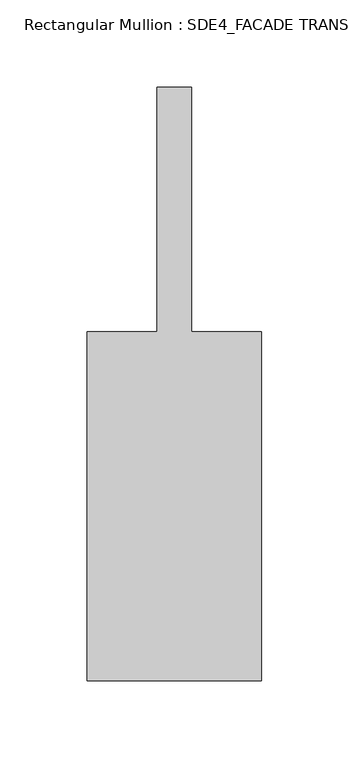
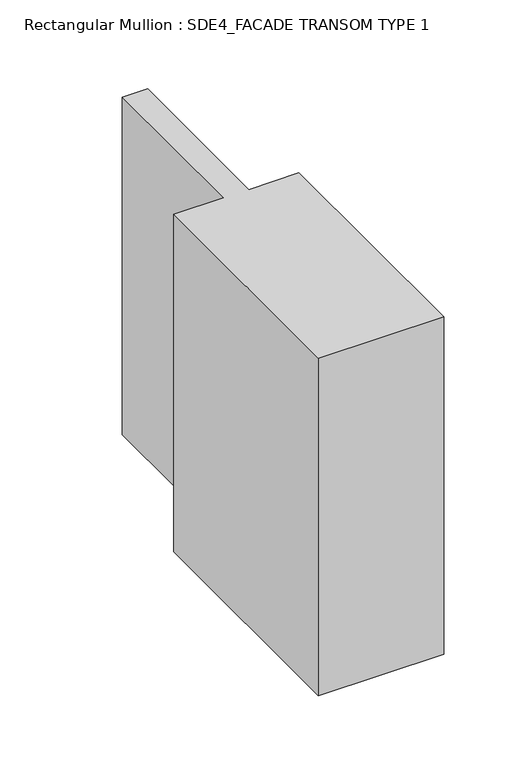
"""IFC4 building model written with IfcOpenShell, lengths in millimetres: member geometry, Rectangular Mullion : SDE4_FACADE TRANSOM TYPE 1."""

from ifc_helpers import new_model, si_unit, frame, origin, place, context, project, spatial, polyline, outline, extrude, source, transform, mapped, element, save


def rectangular_mullion_sde4_facade_transom_type_1_73f302f2(model_context):
    return source(origin(), model_context, "Body", "SweptSolid", [
        extrude(outline(polyline([(50.0, -132.5), (-50.0, -132.5), (-50.0, 67.5), (-10.0, 67.5), (-10.0, 207.5), (10.0, 207.5), (10.0, 67.5), (50.0, 67.5), (50.0, -132.5)])), frame((0.0, 0.0, -284.7600538), z_axis=(0.0, 0.0, 1.0), x_axis=(1.0, 0.0, 0.0)), (0.0, 0.0, 1.0), 284.7600538),
    ])


if __name__ == "__main__":
    model = new_model("IFC4")
    model_context = context("Model", 3, world=origin())
    ifc_project = project(units=[si_unit("LENGTHUNIT", "METRE", prefix="MILLI")], contexts=[model_context])
    site = spatial("IfcSite", under=ifc_project)
    building = spatial("IfcBuilding", under=site)
    placement = place(None, origin())
    rectangular_mullion_sde4_facade_transom_type_1_shape = rectangular_mullion_sde4_facade_transom_type_1_73f302f2(model_context)
    element("IfcMember", 1, ObjectType="Rectangular Mullion : SDE4_FACADE TRANSOM TYPE 1", at=placement, inside=building, context=model_context, shape_type="MappedRepresentation", body=[
        mapped(rectangular_mullion_sde4_facade_transom_type_1_shape, transform((0.0, 0.0, 0.0), x_axis=(1.0, 0.0, 0.0), y_axis=(0.0, 1.0, 0.0), z_axis=(0.0, 0.0, 1.0))),
    ])
    save(model, "model.ifc")

# Revit data of these elements
# Type "Rectangular Mullion : SDE4_FACADE TRANSOM TYPE 1"
#   built-in parameter 1007322 = 1.11549 (stored number, unit not read)
#   built-in parameter 1007321 = 0.164042 (stored number, unit not read)
#   built-in parameter 1007320 = 0.164042 (stored number, unit not read)
